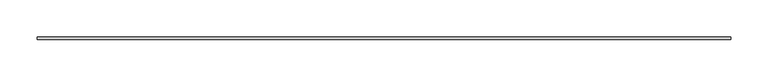
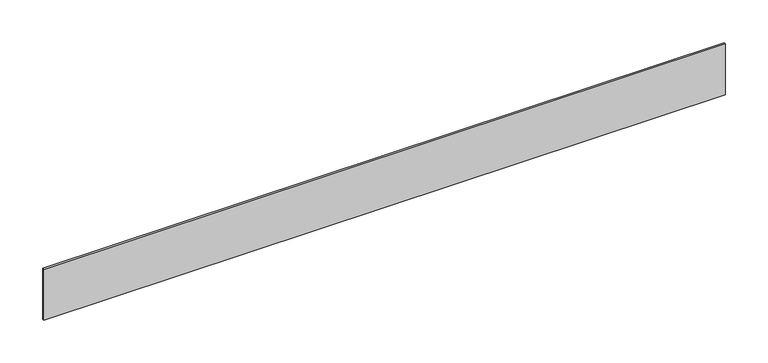
"""IFC4 building model written with IfcOpenShell, lengths in millimetres: proxy geometry, Generic Models 6:Generic Models 2:318829:Generic Models 2:318829 : Generic Models 6:Generic Models 2:318829:17 : Generic Models 6:Generic Models 2:318829:Generic Models 2:318829 : Generic Models 6:Generic Models 2:318829:300683."""

from ifc_helpers import new_model, si_unit, frame, origin, place, context, project, spatial, polyline, outline, extrude, source, transform, mapped, element, save


def generic_models_f2dcbbd7(model_context):
    return source(origin(), model_context, "Body", "SweptSolid", [
        extrude(outline(polyline([(593679.9536635, -578997.343279), (593679.9536635, -579000.518279), (592755.4242239, -579000.518279), (592755.4242239, -578997.343279), (593679.9536635, -578997.343279)])), frame((0.0, 0.0, 3.3705197), z_axis=(0.0, 0.0, 1.0), x_axis=(1.0, 0.0, 0.0)), (0.0, 0.0, 1.0), 72.8294803),
    ])


if __name__ == "__main__":
    model = new_model("IFC4")
    model_context = context("Model", 3, world=origin())
    ifc_project = project(units=[si_unit("LENGTHUNIT", "METRE", prefix="MILLI")], contexts=[model_context])
    site = spatial("IfcSite", under=ifc_project)
    building = spatial("IfcBuilding", under=site)
    placement = place(None, origin())
    generic_models_shape = generic_models_f2dcbbd7(model_context)
    element("IfcBuildingElementProxy", 1, Name="Generic Models 6:Generic Models 2:318829:Generic Models 2:318829 : Generic Models 6:Generic Models 2:318829:17 : Generic Models 6:Generic Models 2:318829:Generic Models 2:318829 : Generic Models 6:Generic Models 2:318829:300683", ObjectType="Generic Models 6:Generic Models 2:318829:Generic Models 2:318829 : Generic Models 6:Generic Models 2:318829:17 : Generic Models 6:Generic Models 2:318829:Generic Models 2:318829 : Generic Models 6:Generic Models 2:318829:300683", at=placement, inside=building, context=model_context, shape_type="MappedRepresentation", body=[
        mapped(generic_models_shape, transform((0.0, 0.0, 0.0), x_axis=(1.0, 0.0, 0.0), y_axis=(0.0, 1.0, 0.0), z_axis=(0.0, 0.0, 1.0))),
    ])
    save(model, "model.ifc")

# Revit data of these elements
# Type "Generic Models 6:Generic Models 2:318829:Generic Models 2:318829 : Generic Models 6:Generic Models 2:318829:17 : Generic Models 6:Generic Models 2:318829:Generic Models 2:318829 : Generic Models 6:Generic Models 2:318829:300683"
#   NameOverride = "Generic Models 6:Generic Models 2:318829:Generic Models 2:318829 : Generic Models 6:Generic Models 2:318829:300683"
#   ObjectTypeOverride = "Generic Models 2:318829 : Generic Models 6:Generic Models 2:318829"
#   Reference = "Generic Models 2"
#   Tag = "300683"
# Element 1 (IfcBuildingElementProxy, "Generic Models 6:Generic Models 2:318829:Generic Models 2:318829 : Generic Models 6:Generic Models 2:318829:17 : Generic Models 6:Generic Models 2:318829:Generic Models 2:318829 : Generic Models 6:Generic Models 2:318829:300683")
#   Materials on its faces: "ALUM. BASE TRIM"
# Materials
#   "ALUM. BASE TRIM": class "Generic", colour RGB 120 120 120, transparency 0, Cost = 0
